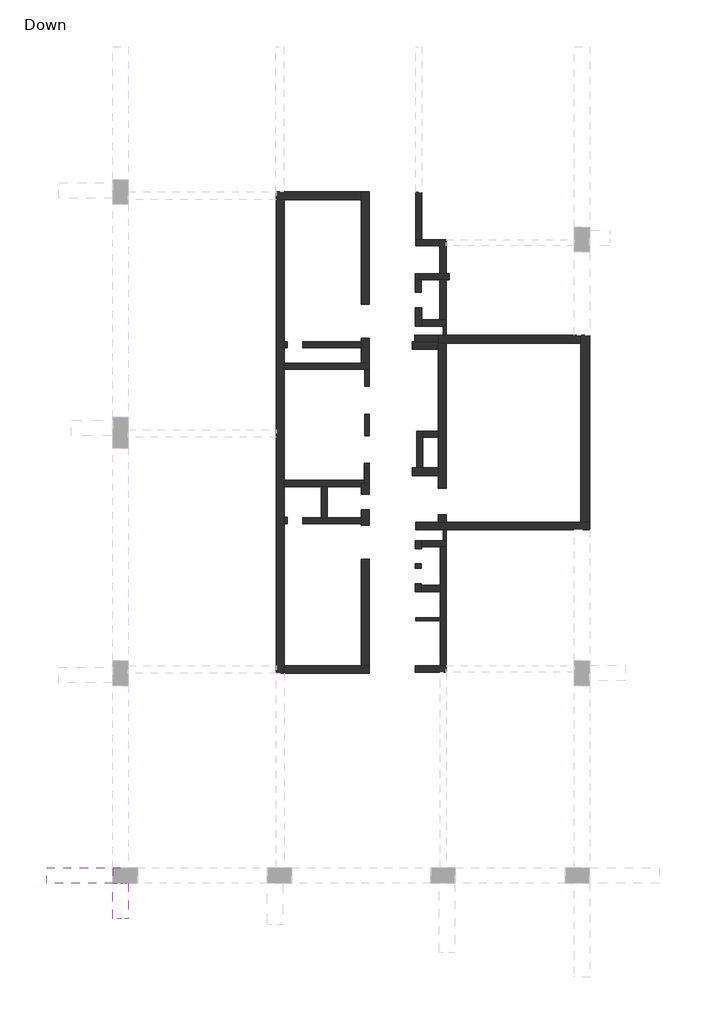
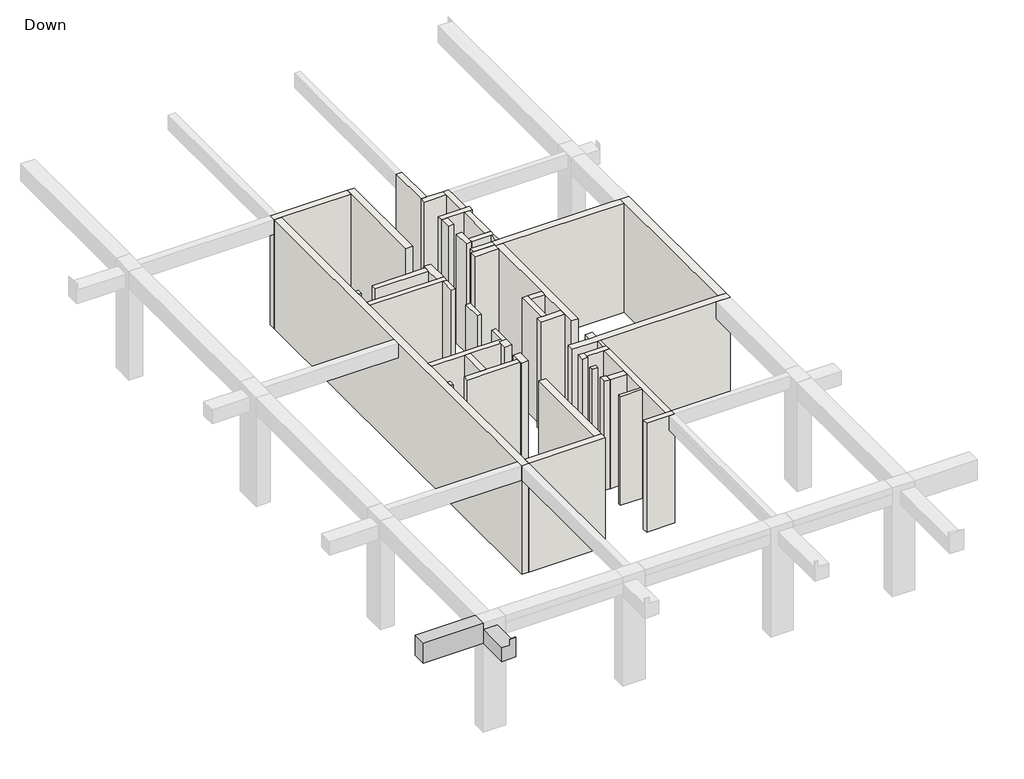
# One storey, part 1 of 2: 46 walls, 2 beams.
# Revit data of these elements (continued)
# Element 31 (IfcWall, "20") (continued)
#   Comments = ""
#   Mark = "W40"
#   SOFiSTiK_EdgeZones = "W40"
#   SOFiSTiK_AMG_Comments = ""
#   Top Offset = 0 cm
#   Base Offset = 0 cm
#   wall height = 412.5 cm
#   SOFiSTiK_AMG_Scheduled = yes
#   SOFiSTiK_AMG_Adjusted = yes
#   Phase Created = New Construction
#   Base Constraint = Down
#   Top Constraint = Typical Floor
#   Materials on its faces: "Concrete"
# Element 32 (IfcWall, "20")
#   Comments = ""
#   Mark = "W41"
#   SOFiSTiK_EdgeZones = "W41"
#   SOFiSTiK_AMG_Comments = ""
#   Top Offset = 0 cm
#   Base Offset = 0 cm
#   wall height = 412.5 cm
#   SOFiSTiK_AMG_Scheduled = yes
#   SOFiSTiK_AMG_Adjusted = yes
#   Phase Created = New Construction
#   Base Constraint = Down
#   Top Constraint = Typical Floor
#   Materials on its faces: "Concrete"
# Element 33 (IfcWall, "20")
#   Comments = ""
#   Mark = "W43"
#   SOFiSTiK_EdgeZones = "W43"
#   SOFiSTiK_AMG_Comments = ""
#   Top Offset = 0 cm
#   Base Offset = 0 cm
#   wall height = 412.5 cm
#   SOFiSTiK_AMG_Scheduled = yes
#   SOFiSTiK_AMG_Adjusted = yes
#   Phase Created = New Construction
#   Base Constraint = Down
#   Top Constraint = Typical Floor
#   Materials on its faces: "Concrete"
# Element 34 (IfcWall, "25")
#   Comments = ""
#   Mark = "W1"
#   SOFiSTiK_EdgeZones = "W1"
#   SOFiSTiK_AMG_Comments = ""
#   Top Offset = 0 cm
#   Base Offset = 0 cm
#   wall height = 412.5 cm
#   SOFiSTiK_AMG_Scheduled = yes
#   SOFiSTiK_AMG_Adjusted = yes
#   Phase Created = New Construction
#   Base Constraint = Down
#   Top Constraint = Typical Floor
#   Materials on its faces: "Concrete"
# Element 35 (IfcWall, "25")
#   Comments = ""
#   Mark = "W2"
#   SOFiSTiK_EdgeZones = "W2"
#   SOFiSTiK_AMG_Comments = ""
#   Top Offset = 0 cm
#   Base Offset = 0 cm
#   wall height = 412.5 cm
#   SOFiSTiK_AMG_Scheduled = yes
#   SOFiSTiK_AMG_Adjusted = yes
#   Phase Created = New Construction
#   Base Constraint = Down
#   Top Constraint = Typical Floor
#   Materials on its faces: "Concrete"
# Element 36 (IfcWall, "25")
#   Comments = ""
#   Mark = "W3"
#   SOFiSTiK_EdgeZones = "W3"
#   SOFiSTiK_AMG_Comments = ""
#   Top Offset = 0 cm
#   Base Offset = 0 cm
#   wall height = 412.5 cm
#   SOFiSTiK_AMG_Scheduled = yes
#   SOFiSTiK_AMG_Adjusted = yes
#   Phase Created = New Construction
#   Base Constraint = Down
#   Top Constraint = Typical Floor
#   Materials on its faces: "Concrete"
# Element 37 (IfcWall, "25")
#   Comments = ""
#   Mark = "W4"
#   SOFiSTiK_EdgeZones = "W4"
#   SOFiSTiK_AMG_Comments = ""
#   Top Offset = 0 cm
#   Base Offset = 0 cm
#   wall height = 412.5 cm
#   SOFiSTiK_AMG_Scheduled = yes
#   SOFiSTiK_AMG_Adjusted = yes
#   Phase Created = New Construction
#   Base Constraint = Down
#   Top Constraint = Typical Floor
#   Materials on its faces: "Concrete"
# Element 38 (IfcWall, "25")
#   Comments = ""
#   Mark = "W5"
#   SOFiSTiK_EdgeZones = "W5"
#   SOFiSTiK_AMG_Comments = ""
#   Top Offset = 0 cm
#   Base Offset = 0 cm
#   wall height = 412.5 cm
#   SOFiSTiK_AMG_Scheduled = yes
#   SOFiSTiK_AMG_Adjusted = yes
#   Phase Created = New Construction
#   Base Constraint = Down
#   Top Constraint = Typical Floor
#   Materials on its faces: "Concrete"
# Element 39 (IfcWall, "25")
#   Comments = ""
#   Mark = "W6"
#   SOFiSTiK_EdgeZones = "W6"
#   SOFiSTiK_AMG_Comments = ""
#   Top Offset = 0 cm
#   Base Offset = 0 cm
#   wall height = 412.5 cm
#   SOFiSTiK_AMG_Scheduled = yes
#   SOFiSTiK_AMG_Adjusted = yes
#   Phase Created = New Construction
#   Base Constraint = Down
#   Top Constraint = Typical Floor
#   Materials on its faces: "Concrete"
# Element 40 (IfcWall, "25")
#   Comments = ""
#   Mark = "W7"
#   SOFiSTiK_EdgeZones = "W7"
#   SOFiSTiK_AMG_Comments = ""
#   Top Offset = 0 cm
#   Base Offset = 0 cm
#   wall height = 412.5 cm
#   SOFiSTiK_AMG_Scheduled = yes
#   SOFiSTiK_AMG_Adjusted = yes
#   Phase Created = New Construction
#   Base Constraint = Down
#   Top Constraint = Typical Floor
#   Materials on its faces: "Concrete"
# Element 41 (IfcWall, "25")
#   Comments = ""
#   Mark = "W8"
#   SOFiSTiK_EdgeZones = "W8"
#   SOFiSTiK_AMG_Comments = ""
#   Top Offset = 0 cm
#   Base Offset = 0 cm
#   wall height = 412.5 cm
#   SOFiSTiK_AMG_Scheduled = yes
#   SOFiSTiK_AMG_Adjusted = yes
#   Phase Created = New Construction
#   Base Constraint = Down
#   Top Constraint = Typical Floor
#   Materials on its faces: "Concrete"
# Element 42 (IfcWall, "25")
#   Comments = ""
#   Mark = "W9"
#   SOFiSTiK_EdgeZones = "W9"
#   SOFiSTiK_AMG_Comments = ""
#   Top Offset = 0 cm
#   Base Offset = 0 cm
#   wall height = 412.5 cm
#   SOFiSTiK_AMG_Scheduled = yes
#   SOFiSTiK_AMG_Adjusted = yes
#   Phase Created = New Construction
#   Base Constraint = Down
#   Top Constraint = Typical Floor
#   Materials on its faces: "Concrete"
# Element 43 (IfcWall, "25")
#   Comments = ""
#   Mark = "W10"
#   SOFiSTiK_EdgeZones = "W10"
#   SOFiSTiK_AMG_Comments = ""
#   Top Offset = 0 cm
#   Base Offset = 0 cm
#   wall height = 412.5 cm
#   SOFiSTiK_AMG_Scheduled = yes
#   SOFiSTiK_AMG_Adjusted = yes
#   Phase Created = New Construction
#   Base Constraint = Down
#   Top Constraint = Typical Floor
#   Materials on its faces: "Concrete"
# Element 44 (IfcWall, "25")
#   Comments = ""
#   Mark = "W11"
#   SOFiSTiK_EdgeZones = "W11"
#   SOFiSTiK_AMG_Comments = ""
#   Top Offset = 0 cm
#   Base Offset = 0 cm
#   wall height = 412.5 cm
#   SOFiSTiK_AMG_Scheduled = yes
#   SOFiSTiK_AMG_Adjusted = yes
#   Phase Created = New Construction
#   Base Constraint = Down
#   Top Constraint = Typical Floor
#   Materials on its faces: "Concrete"
# Element 45 (IfcWall, "25")
#   Comments = ""
#   Mark = "W12"
#   SOFiSTiK_EdgeZones = "W12"
#   SOFiSTiK_AMG_Comments = ""
#   Top Offset = 0 cm
#   Base Offset = 0 cm
#   wall height = 412.5 cm
#   SOFiSTiK_AMG_Scheduled = yes
#   SOFiSTiK_AMG_Adjusted = yes
#   Phase Created = New Construction
#   Base Constraint = Down
#   Top Constraint = Typical Floor
#   Materials on its faces: "Concrete"
# Element 46 (IfcWall, "25")
#   Comments = ""
#   Mark = "W13"
#   SOFiSTiK_EdgeZones = "W13"
#   SOFiSTiK_AMG_Comments = ""
#   Top Offset = 0 cm
#   Base Offset = 0 cm
#   wall height = 412.5 cm
#   SOFiSTiK_AMG_Scheduled = yes
#   SOFiSTiK_AMG_Adjusted = yes
#   Phase Created = New Construction
#   Base Constraint = Down
#   Top Constraint = Typical Floor
#   Materials on its faces: "Concrete"
# Element 47 (IfcWall, "25")
#   Comments = ""
#   Mark = "W14"
#   SOFiSTiK_EdgeZones = "W14"
#   SOFiSTiK_AMG_Comments = ""
#   Top Offset = 0 cm
#   Base Offset = 0 cm
#   wall height = 412.5 cm
#   SOFiSTiK_AMG_Scheduled = yes
#   SOFiSTiK_AMG_Adjusted = yes
#   Phase Created = New Construction
#   Base Constraint = Down
#   Top Constraint = Typical Floor
#   Materials on its faces: "Concrete"
# Element 48 (IfcWall, "30")
#   Comments = ""
#   Mark = "W16"
#   SOFiSTiK_EdgeZones = "W16"
#   SOFiSTiK_AMG_Comments = ""
#   Top Offset = 0 cm
#   Base Offset = 0 cm
#   wall height = 412.5 cm
#   SOFiSTiK_AMG_Scheduled = yes
#   SOFiSTiK_AMG_Adjusted = yes
#   Phase Created = New Construction
#   Base Constraint = Down
#   Top Constraint = Typical Floor
#   Materials on its faces: "Concrete"
# Materials
#   "Concrete": class "Concrete", colour RGB 192 192 192, transparency 0, Keynote = "01000", Description = "Cast-in-place concrete", Cost = 0
